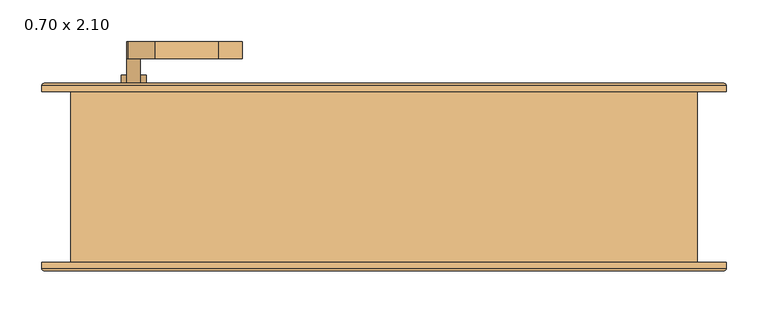
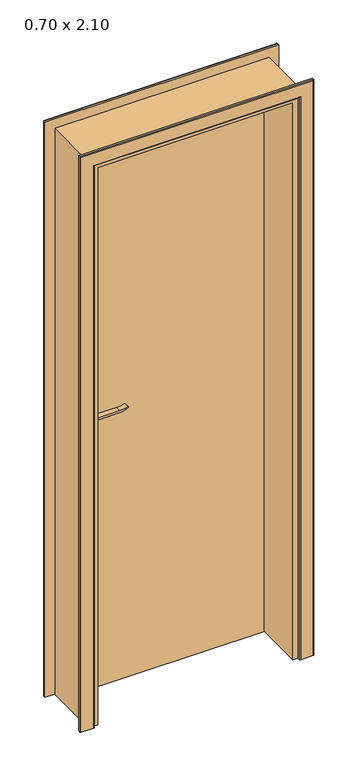
"""IFC4 building model written with IfcOpenShell, lengths in millimetres: door geometry, .CC_ND 300_PORTA SIMPLES DE ABRIR_COM EXTENSÃO : 0.70 x 2.10."""

import ifcopenshell
import ifcopenshell.guid

model = None  # the IFC model being written
_history = None  # IfcOwnerHistory: only IFC2X3 demands one
_inside = {}  # id of a spatial element -> (the spatial element, [elements in it])
_under = {}  # id of a project, library or spatial element -> (it, [spatial elements below it])
_declared = {}  # id of a project -> (the project, [libraries it declares])
_typed = {}  # id of a type object -> (the type object, [elements of that type])
_made_of = {}  # id of a material, layer set ... -> (it, [elements and type objects made of it])


def new_model(schema):
    """Start an empty IFC model of exactly this schema.

    Asked for "IFC4X3", IfcOpenShell would pick the latest addendum, in which some entities
    have other attributes; the version numbers below select the first issue.
    IFC2X3 requires an IfcOwnerHistory on every rooted entity: one is made here for all.
    """
    global model, _history
    if schema == "IFC4X3":
        model = ifcopenshell.file(schema_version=(4, 3, 0, 0))
    else:
        model = ifcopenshell.file(schema=schema)
    _inside.clear()
    _under.clear()
    _declared.clear()
    _typed.clear()
    _made_of.clear()
    _history = None
    if model.schema == "IFC2X3":
        org = make("IfcOrganization", Name="unknown")
        user = make(
            "IfcPersonAndOrganization",
            ThePerson=make("IfcPerson", FamilyName="unknown"),
            TheOrganization=org,
        )
        app = make(
            "IfcApplication",
            ApplicationDeveloper=org,
            Version="unknown",
            ApplicationFullName="unknown",
            ApplicationIdentifier="unknown",
        )
        _history = make(
            "IfcOwnerHistory",
            OwningUser=user,
            OwningApplication=app,
            ChangeAction="ADDED",
            CreationDate=0,
        )
    return model


def make(cls, **values):
    """One entity of the class cls with the attributes given. An attribute that is None is left unset."""
    return model.create_entity(
        cls, **{name: value for name, value in values.items() if value is not None}
    )


def rooted(cls, **values):
    """An entity with a GlobalId (a new one), such as an element, a storey or a relation."""
    return make(cls, GlobalId=ifcopenshell.guid.new(), OwnerHistory=_history, **values)


def si_unit(unit_type, name, prefix=None):
    """IfcSIUnit, for example si_unit("LENGTHUNIT", "METRE", prefix="MILLI")."""
    return make("IfcSIUnit", UnitType=unit_type, Prefix=prefix, Name=name)


def assignment(units):
    """IfcUnitAssignment: the units of a project."""
    return None if units is None else make("IfcUnitAssignment", Units=units)


def point(xyz):
    """IfcCartesianPoint."""
    return None if xyz is None else make("IfcCartesianPoint", Coordinates=xyz)


def direction(xyz):
    """IfcDirection."""
    return None if xyz is None else make("IfcDirection", DirectionRatios=xyz)


def frame(location, z_axis=None, x_axis=None):
    """IfcAxis2Placement3D, a coordinate frame: its origin and axes. An axis left out is left unset."""
    return make(
        "IfcAxis2Placement3D",
        Location=point(location),
        Axis=direction(z_axis),
        RefDirection=direction(x_axis),
    )


def frame_2d(location, x_axis=None):
    """IfcAxis2Placement2D, a coordinate frame in the plane: its origin and x axis."""
    return make(
        "IfcAxis2Placement2D", Location=point(location), RefDirection=direction(x_axis)
    )


def origin():
    """The frame at (0, 0, 0) with its axes left unset."""
    return frame((0.0, 0.0, 0.0))


def origin_with_axes():
    """The frame at (0, 0, 0) with the z axis (0, 0, 1) and the x axis (1, 0, 0) written out."""
    return frame((0.0, 0.0, 0.0), z_axis=(0.0, 0.0, 1.0), x_axis=(1.0, 0.0, 0.0))


def place(relative_to, where):
    """IfcLocalPlacement: puts the frame where relative to a parent placement (None: the world)."""
    return make(
        "IfcLocalPlacement", PlacementRelTo=relative_to, RelativePlacement=where
    )


def context(
    kind, dimensions, precision=None, world=None, true_north=None, identifier=None
):
    """IfcGeometricRepresentationContext, for example the 3D "Model" context."""
    return make(
        "IfcGeometricRepresentationContext",
        ContextIdentifier=identifier,
        ContextType=kind,
        CoordinateSpaceDimension=dimensions,
        Precision=precision,
        WorldCoordinateSystem=world,
        TrueNorth=true_north,
    )


def project(units=None, contexts=None):
    """IfcProject with its units and contexts."""
    return rooted(
        "IfcProject",
        Name="project",
        RepresentationContexts=contexts,
        UnitsInContext=assignment(units),
    )


def spatial(cls, under=None, at=None, **own):
    """A site, building, storey or space (cls), placed at a placement, below another one or the project."""
    s = rooted(cls, ObjectPlacement=at, **own)
    if under is not None:
        _under.setdefault(under.id(), (under, []))[1].append(s)
    return s


def polyline(points):
    """IfcPolyline through the points."""
    return make("IfcPolyline", Points=[point(p) for p in points])


def circle_curve(where, radius):
    """IfcCircle in the frame where."""
    return make("IfcCircle", Position=where, Radius=radius)


def ellipse_curve(where, semi_axis1, semi_axis2):
    """IfcEllipse in the frame where."""
    return make(
        "IfcEllipse", Position=where, SemiAxis1=semi_axis1, SemiAxis2=semi_axis2
    )


def trimmed(basis, trim1, trim2, sense, master):
    """IfcTrimmedCurve: the piece of a basis curve between two trims."""
    return make(
        "IfcTrimmedCurve",
        BasisCurve=basis,
        Trim1=trim1,
        Trim2=trim2,
        SenseAgreement=sense,
        MasterRepresentation=master,
    )


def segment(curve, same_sense, transition):
    """IfcCompositeCurveSegment."""
    return make(
        "IfcCompositeCurveSegment",
        Transition=transition,
        SameSense=same_sense,
        ParentCurve=curve,
    )


def composite_curve(segments, self_intersect=None):
    """IfcCompositeCurve: segments joined end to end."""
    return make("IfcCompositeCurve", Segments=segments, SelfIntersect=self_intersect)


def outline(outer, holes=None, kind="AREA"):
    """IfcArbitraryClosedProfileDef: a profile drawn as a closed curve; with holes, ...WithVoids."""
    if holes is None:
        return make("IfcArbitraryClosedProfileDef", ProfileType=kind, OuterCurve=outer)
    return make(
        "IfcArbitraryProfileDefWithVoids",
        ProfileType=kind,
        OuterCurve=outer,
        InnerCurves=holes,
    )


def extrude(swept, where, along, depth):
    """IfcExtrudedAreaSolid: the profile swept, set in the frame where, extruded along a direction by depth."""
    return make(
        "IfcExtrudedAreaSolid",
        SweptArea=swept,
        Position=where,
        ExtrudedDirection=direction(along),
        Depth=depth,
    )


def faces_of(points, faces, orient=None, outer=None):
    """IfcFace entities. A face is a list of loops; a loop is a list of indices into points, from 0.

    orient and outer hold one flag for each loop. By default every Orientation is true, the
    first loop of a face is its IfcFaceOuterBound and the others are IfcFaceBound.
    """
    made = []
    for i, loops in enumerate(faces):
        bounds = []
        for j, loop in enumerate(loops):
            is_outer = j == 0 if outer is None else outer[i][j]
            bounds.append(
                make(
                    "IfcFaceOuterBound" if is_outer else "IfcFaceBound",
                    Bound=make("IfcPolyLoop", Polygon=[points[k] for k in loop]),
                    Orientation=True if orient is None else orient[i][j],
                )
            )
        made.append(make("IfcFace", Bounds=bounds))
    return made


def faceted_brep(points, faces, orient=None, outer=None, voids=None):
    """IfcFacetedBrep: a solid bounded by flat faces; with voids (closed shells), ...WithVoids."""
    shared = [point(p) for p in points]
    hull = make("IfcClosedShell", CfsFaces=faces_of(shared, faces, orient, outer))
    if voids is None:
        return make("IfcFacetedBrep", Outer=hull)
    return make(
        "IfcFacetedBrepWithVoids",
        Outer=hull,
        Voids=[
            make(cls, CfsFaces=faces_of(shared, fs, o, b)) for cls, fs, o, b in voids
        ],
    )


def shape(context_of_items, identifier, shape_type, items):
    """IfcShapeRepresentation: the items that make up one representation, for example the "Body"."""
    return make(
        "IfcShapeRepresentation",
        ContextOfItems=context_of_items,
        RepresentationIdentifier=identifier,
        RepresentationType=shape_type,
        Items=items,
    )


def source(mapping_origin, context_of_items, identifier, shape_type, items):
    """IfcRepresentationMap: a shape defined once, which mapped items show again and again."""
    return make(
        "IfcRepresentationMap",
        MappingOrigin=mapping_origin,
        MappedRepresentation=shape(context_of_items, identifier, shape_type, items),
    )


def transform(
    local_origin,
    x_axis=None,
    y_axis=None,
    z_axis=None,
    scale=None,
    scale2=None,
    scale3=None,
    uniform=True,
):
    """IfcCartesianTransformationOperator3D, or its non-uniform kind. x_axis, y_axis, z_axis: its Axis1, 2, 3."""
    if uniform:
        return make(
            "IfcCartesianTransformationOperator3D",
            Axis1=direction(x_axis),
            Axis2=direction(y_axis),
            LocalOrigin=point(local_origin),
            Scale=scale,
            Axis3=direction(z_axis),
        )
    return make(
        "IfcCartesianTransformationOperator3DnonUniform",
        Axis1=direction(x_axis),
        Axis2=direction(y_axis),
        LocalOrigin=point(local_origin),
        Scale=scale,
        Axis3=direction(z_axis),
        Scale2=scale2,
        Scale3=scale3,
    )


def mapped(mapping_source, mapping_target):
    """IfcMappedItem: shows the shape of a source again, moved by a transform."""
    return make(
        "IfcMappedItem", MappingSource=mapping_source, MappingTarget=mapping_target
    )


def made_of(thing, what):
    """Note that an element or type object is made of a material, layer set ...; save() writes the relation."""
    if what is not None:
        _made_of.setdefault(what.id(), (what, []))[1].append(thing)
    return thing


def element(
    cls,
    number,
    at=None,
    inside=None,
    cuts=None,
    type_object=None,
    material=None,
    context=None,
    identifier="Body",
    shape_type=None,
    held_by="IfcProductDefinitionShape",
    body=None,
    shapes=None,
    **own,
):
    """One element of the class cls, such as IfcWall. Its Tag is "e" and its number.

    at: its placement. inside: the storey or other place that contains it. cuts: it is an
    opening in that element (IfcRelVoidsElement). A single representation is given by context,
    identifier, shape_type and body (its items); several are given by shapes. held_by: the class
    of the entity that holds the representations. save() writes the other relations.
    """
    e = rooted(cls, Tag="e%d" % number, ObjectPlacement=at, **own)
    if body is not None:
        shapes = [shape(context, identifier, shape_type, body)]
    if shapes is not None:
        e.Representation = make(held_by, Representations=shapes)
    if inside is not None:
        _inside.setdefault(inside.id(), (inside, []))[1].append(e)
    if cuts is not None:
        rooted(
            "IfcRelVoidsElement", RelatingBuildingElement=cuts, RelatedOpeningElement=e
        )
    if type_object is not None:
        _typed.setdefault(type_object.id(), (type_object, []))[1].append(e)
    return made_of(e, material)


def aggregate(whole, parts):
    """IfcRelAggregates: a whole, such as a stair, and the parts it consists of."""
    return rooted("IfcRelAggregates", RelatingObject=whole, RelatedObjects=parts)


def save(model, path):
    """Write the relations noted so far, then the file.

    IfcRelAggregates (storeys below a building ...), IfcRelContainedInSpatialStructure (elements
    in a storey), IfcRelDefinesByType, IfcRelAssociatesMaterial and IfcRelDeclares: one each for
    every whole, place, type object, material and project.
    """
    for whole, parts in _under.values():
        aggregate(whole, parts)
    for where, things in _inside.values():
        rooted(
            "IfcRelContainedInSpatialStructure",
            RelatedElements=things,
            RelatingStructure=where,
        )
    for kind, things in _typed.values():
        rooted("IfcRelDefinesByType", RelatedObjects=things, RelatingType=kind)
    for what, things in _made_of.values():
        rooted("IfcRelAssociatesMaterial", RelatedObjects=things, RelatingMaterial=what)
    for by, libraries in _declared.values():
        rooted("IfcRelDeclares", RelatingContext=by, RelatedDefinitions=libraries)
    model.write(path)


def plane_surface(at):
    """IfcPlane: the flat surface through the origin of the frame at, square to its z axis."""
    return make("IfcPlane", Position=at)


def cylinder_surface(at, radius):
    """IfcCylindricalSurface: all points at the distance radius from the z axis of the frame at."""
    return make("IfcCylindricalSurface", Position=at, Radius=radius)


def advanced_brep(points, edges, surfaces, faces):
    """IfcAdvancedBrep: a solid bounded by faces that lie on surfaces and meet in shared edges.

    An edge is (start, end): straight between two places in points (the first is 0);
    or (start, end, curve); or (start, end, curve, False) where it runs against its curve.
    A face is (place in surfaces, loops), or (place, loops, False) where it looks against
    its surface's normal. A loop lists edges by number (the first is 1), with a minus sign
    where the edge is run from its end to its start. The first loop is the outer one.
    """
    corners = [point(p) for p in points]
    vertices = [make("IfcVertexPoint", VertexGeometry=c) for c in corners]
    made = []
    for start, end, *more in edges:
        made.append(
            make(
                "IfcEdgeCurve",
                EdgeStart=vertices[start],
                EdgeEnd=vertices[end],
                EdgeGeometry=more[0] if more else make("IfcPolyline", Points=[corners[start], corners[end]]),
                SameSense=more[1] if len(more) > 1 else True,
            )
        )
    hull = []
    for where, loops, *sense in faces:
        bounds = []
        for j, loop in enumerate(loops):
            ring = [make("IfcOrientedEdge", EdgeElement=made[abs(k) - 1], Orientation=k > 0) for k in loop]
            bounds.append(
                make(
                    "IfcFaceOuterBound" if j == 0 else "IfcFaceBound",
                    Bound=make("IfcEdgeLoop", EdgeList=ring),
                    Orientation=True,
                )
            )
        hull.append(make("IfcAdvancedFace", Bounds=bounds, FaceSurface=surfaces[where], SameSense=sense[0] if sense else True))
    return make("IfcAdvancedBrep", Outer=make("IfcClosedShell", CfsFaces=hull))


def door_0_70_x_2_10_01854108(model_context):
    return source(origin(), model_context, "Body", "SolidModel", [
        extrude(outline(composite_curve([segment(trimmed(circle_curve(frame_2d((964.5, -300.0)), 15.0), [point((964.5, -285.0))], [point((964.5, -315.0))], False, "CARTESIAN"), True, "CONTINUOUS"), segment(trimmed(circle_curve(frame_2d((964.5, -300.0)), 15.0), [point((964.5, -315.0))], [point((964.5, -285.0))], False, "CARTESIAN"), True, "CONTINUOUS")], self_intersect=False)), frame((0.0, 127.9, 0.0), z_axis=(0.0, 1.0, 0.0), x_axis=(0.0, 0.0, 1.0)), (0.0, 0.0, 1.0), 10.0),
        extrude(outline(composite_curve([segment(trimmed(circle_curve(frame_2d((964.5, -300.0)), 15.0), [point((964.5, -285.0))], [point((964.5, -315.0))], False, "CARTESIAN"), True, "CONTINUOUS"), segment(trimmed(circle_curve(frame_2d((964.5, -300.0)), 15.0), [point((964.5, -315.0))], [point((964.5, -285.0))], False, "CARTESIAN"), True, "CONTINUOUS")], self_intersect=False)), frame((0.0, 67.9, 0.0), z_axis=(0.0, 1.0, 0.0), x_axis=(0.0, 0.0, 1.0)), (0.0, 0.0, 1.0), 10.0),
        extrude(outline(composite_curve([segment(trimmed(circle_curve(frame_2d((1024.5, -300.0)), 8.0), [point((1029.1523287, -306.5081363))], [point((1024.5, -292.0))], False, "CARTESIAN"), True, "CONTINUOUS"), segment(trimmed(circle_curve(frame_2d((1019.3738613, -274.6138099)), 18.1261387), [point((1024.5, -292.0))], [point((1037.5, -274.6138099))], True, "CARTESIAN"), True, "CONTINUOUS"), segment(polyline([(1037.5, -274.6138099), (1037.5, -198.3564091)]), True, "CONTINUOUS"), segment(trimmed(circle_curve(frame_2d((1096.7709207, -201.9396612)), 59.3791355), [point((1037.5, -198.3564091))], [point((1046.7135558, -170.0))], False, "CARTESIAN"), True, "CONTINUOUS"), segment(polyline([(1046.7135558, -170.0), (1049.5, -170.0)]), True, "CONTINUOUS"), segment(trimmed(circle_curve(frame_2d((1127.7850638, -198.4227909)), 83.2850902), [point((1049.5, -170.0))], [point((1044.5, -198.3564091))], True, "CARTESIAN"), True, "CONTINUOUS"), segment(polyline([(1044.5, -198.3564091), (1044.5, -274.6325667)]), True, "CONTINUOUS"), segment(trimmed(circle_curve(frame_2d((1007.2555521, -276.3324871)), 37.2832219), [point((1044.5, -274.6325667))], [point((1029.1523287, -306.5081363))], False, "CARTESIAN"), True, "CONTINUOUS")], self_intersect=False)), frame((0.0, 157.9, 0.0), z_axis=(0.0, 1.0, 0.0), x_axis=(0.0, 0.0, 1.0)), (0.0, 0.0, 1.0), 20.0),
        extrude(outline(composite_curve([segment(trimmed(circle_curve(frame_2d((1019.3738682, -274.6138122)), 18.1261318), [point((1024.4999903, -292.0))], [point((1037.5, -274.6138122))], True, "CARTESIAN"), True, "CONTINUOUS"), segment(polyline([(1037.5, -274.6138122), (1037.5, -198.3564091)]), True, "CONTINUOUS"), segment(trimmed(circle_curve(frame_2d((1096.7709207, -201.9396612)), 59.3791355), [point((1037.5, -198.3564091))], [point((1046.7135558, -170.0))], False, "CARTESIAN"), True, "CONTINUOUS"), segment(polyline([(1046.7135558, -170.0), (1049.5, -170.0)]), True, "CONTINUOUS"), segment(trimmed(circle_curve(frame_2d((1127.7850638, -198.4227909)), 83.2850902), [point((1049.5, -170.0))], [point((1044.5, -198.3564091))], True, "CARTESIAN"), True, "CONTINUOUS"), segment(polyline([(1044.5, -198.3564091), (1044.5, -274.6325667)]), True, "CONTINUOUS"), segment(trimmed(circle_curve(frame_2d((1007.2555521, -276.3324871)), 37.2832219), [point((1044.5, -274.6325667))], [point((1029.1523287, -306.5081363))], False, "CARTESIAN"), True, "CONTINUOUS"), segment(trimmed(circle_curve(frame_2d((1024.5, -300.0)), 8.0), [point((1029.1523287, -306.5081363))], [point((1024.4999903, -292.0))], False, "CARTESIAN"), True, "CONTINUOUS")], self_intersect=False)), frame((0.0, 27.9, 0.0), z_axis=(0.0, 1.0, 0.0), x_axis=(0.0, 0.0, 1.0)), (0.0, 0.0, 1.0), 20.0),
        extrude(outline(composite_curve([segment(trimmed(circle_curve(frame_2d((1024.5, -300.0)), 8.0), [point((1024.5, -292.0))], [point((1024.5, -308.0))], False, "CARTESIAN"), True, "CONTINUOUS"), segment(trimmed(circle_curve(frame_2d((1024.5, -300.0)), 8.0), [point((1024.5, -308.0))], [point((1024.5, -292.0))], False, "CARTESIAN"), True, "CONTINUOUS")], self_intersect=False)), frame((0.0, 127.9, 0.0), z_axis=(0.0, 1.0, 0.0), x_axis=(0.0, 0.0, 1.0)), (0.0, 0.0, 1.0), 30.0),
        extrude(outline(composite_curve([segment(trimmed(circle_curve(frame_2d((1024.5, -300.0)), 8.0), [point((1024.5, -292.0))], [point((1024.5, -308.0))], False, "CARTESIAN"), True, "CONTINUOUS"), segment(trimmed(circle_curve(frame_2d((1024.5, -300.0)), 8.0), [point((1024.5, -308.0))], [point((1024.5, -292.0))], False, "CARTESIAN"), True, "CONTINUOUS")], self_intersect=False)), frame((0.0, 47.9, 0.0), z_axis=(0.0, 1.0, 0.0), x_axis=(0.0, 0.0, 1.0)), (0.0, 0.0, 1.0), 30.0),
        extrude(outline(composite_curve([segment(trimmed(circle_curve(frame_2d((954.5, -300.0)), 25.0), [point((954.5, -325.0))], [point((954.5, -275.0))], False, "CARTESIAN"), True, "CONTINUOUS"), segment(polyline([(954.5, -275.0), (1024.5, -275.0)]), True, "CONTINUOUS"), segment(trimmed(circle_curve(frame_2d((1024.5, -300.0)), 25.0), [point((1024.5, -275.0))], [point((1024.5, -325.0))], False, "CARTESIAN"), True, "CONTINUOUS"), segment(polyline([(1024.5, -325.0), (954.5, -325.0)]), True, "CONTINUOUS")], self_intersect=False)), frame((0.0, 117.9, 0.0), z_axis=(0.0, 1.0, 0.0), x_axis=(0.0, 0.0, 1.0)), (0.0, 0.0, 1.0), 10.0),
        extrude(outline(composite_curve([segment(trimmed(circle_curve(frame_2d((954.5, -300.0)), 25.0), [point((954.5, -325.0))], [point((954.5, -275.0))], False, "CARTESIAN"), True, "CONTINUOUS"), segment(polyline([(954.5, -275.0), (1024.5, -275.0)]), True, "CONTINUOUS"), segment(trimmed(circle_curve(frame_2d((1024.5, -300.0)), 25.0), [point((1024.5, -275.0))], [point((1024.5, -325.0))], False, "CARTESIAN"), True, "CONTINUOUS"), segment(polyline([(1024.5, -325.0), (954.5, -325.0)]), True, "CONTINUOUS")], self_intersect=False)), frame((0.0, 77.9, 0.0), z_axis=(0.0, 1.0, 0.0), x_axis=(0.0, 0.0, 1.0)), (0.0, 0.0, 1.0), 10.0),
        advanced_brep(
        [(-410.0, 117.9, 0.0), (-410.0, 124.9, 0.0), (-407.0, 127.9, 0.0), (-363.0, 127.9, 0.0), (-360.0, 124.9, 0.0), (-360.0, 117.9, 0.0), (-360.0, 117.9, 2085.0), (360.0, 117.9, 2085.0), (360.0, 117.9, 0.0), (410.0, 117.9, 0.0), (410.0, 117.9, 2135.0), (-410.0, 117.9, 2135.0), (-360.0, 124.9, 2085.0), (-363.0, 127.9, 2088.0), (-407.0, 127.9, 2132.0), (407.0, 127.9, 2132.0), (407.0, 127.9, 0.0), (363.0, 127.9, 0.0), (363.0, 127.9, 2088.0), (-410.0, 124.9, 2135.0), (410.0, 124.9, 0.0), (410.0, 124.9, 2135.0), (360.0, 124.9, 0.0), (360.0, 124.9, 2085.0)],
        [
            (0, 1),
            (1, 2, circle_curve(frame((-407.0, 124.9, 0.0), z_axis=(0.0, 0.0, -1.0), x_axis=(1.0, 0.0, 0.0)), 3.0)),
            (2, 3),
            (3, 4, circle_curve(frame((-363.0, 124.9, 0.0), z_axis=(0.0, 0.0, -1.0), x_axis=(1.0, 0.0, 0.0)), 3.0)),
            (4, 5),
            (5, 0),
            (5, 6),
            (6, 7),
            (7, 8),
            (8, 9),
            (9, 10),
            (10, 11),
            (11, 0),
            (4, 12),
            (12, 6),
            (3, 13),
            (13, 12, ellipse_curve(frame((-363.0, 124.9, 2088.0), z_axis=(-0.7071067811865475, 0.0, -0.7071067811865475), x_axis=(0.7071067811865474, 0.0, -0.7071067811865476)), 4.2426407, 3.0)),
            (2, 14),
            (14, 15),
            (15, 16),
            (16, 17),
            (17, 18),
            (18, 13),
            (1, 19),
            (19, 14, ellipse_curve(frame((-407.0, 124.9, 2132.0), z_axis=(-0.7071067811865475, 0.0, -0.7071067811865475), x_axis=(0.7071067811865474, 0.0, -0.7071067811865476)), 4.2426407, 3.0)),
            (11, 19),
            (9, 20),
            (20, 21),
            (21, 10),
            (8, 22),
            (22, 17, circle_curve(frame((363.0, 124.9, 0.0), z_axis=(0.0, 0.0, -1.0), x_axis=(-1.0, 0.0, 0.0)), 3.0)),
            (16, 20, circle_curve(frame((407.0, 124.9, 0.0), z_axis=(0.0, 0.0, -1.0), x_axis=(-1.0, 0.0, 0.0)), 3.0)),
            (23, 22),
            (7, 23),
            (23, 18, ellipse_curve(frame((363.0, 124.9, 2088.0), z_axis=(0.7071067811865475, 0.0, -0.7071067811865475), x_axis=(0.7071067811865474, 0.0, 0.7071067811865476)), 4.2426407, 3.0)),
            (15, 21, ellipse_curve(frame((407.0, 124.9, 2132.0), z_axis=(0.7071067811865475, 0.0, -0.7071067811865475), x_axis=(0.7071067811865474, 0.0, 0.7071067811865476)), 4.2426407, 3.0)),
            (12, 23),
            (21, 19),
        ],
        [
            plane_surface(frame((-360.0, 117.9, 0.0), z_axis=(0.0, 0.0, -1.0), x_axis=(0.0, -1.0, 0.0))),
            plane_surface(frame((-410.0, 117.9, 0.0), z_axis=(0.0, -1.0, 0.0), x_axis=(0.0, 0.0, 1.0))),
            plane_surface(frame((-360.0, 117.9, 0.0), z_axis=(1.0, 0.0, 0.0), x_axis=(0.0, 0.0, 1.0))),
            cylinder_surface(frame((-363.0, 124.9, 0.0), z_axis=(0.0, 0.0, -1.0), x_axis=(1.0, 0.0, 0.0)), 3.0),
            plane_surface(frame((-363.0, 127.9, 0.0), z_axis=(0.0, 1.0, 0.0), x_axis=(0.0, 0.0, 1.0))),
            cylinder_surface(frame((-407.0, 124.9, 0.0), z_axis=(0.0, 0.0, -1.0), x_axis=(1.0, 0.0, 0.0)), 3.0),
            plane_surface(frame((-410.0, 124.9, 0.0), z_axis=(-1.0, 0.0, 0.0), x_axis=(0.0, 0.0, 1.0))),
            plane_surface(frame((410.0, 124.9, 2135.0), z_axis=(1.0, 0.0, 0.0), x_axis=(0.0, 0.0, -1.0))),
            plane_surface(frame((360.0, 117.9, 0.0), z_axis=(0.0, 0.0, -1.0), x_axis=(0.0, -1.0, 0.0))),
            plane_surface(frame((360.0, 117.9, 2085.0), z_axis=(-1.0, 0.0, 0.0), x_axis=(0.0, 0.0, -1.0))),
            cylinder_surface(frame((363.0, 124.9, 2085.0), z_axis=(0.0, 0.0, 1.0), x_axis=(-1.0, 0.0, 0.0)), 3.0),
            cylinder_surface(frame((407.0, 124.9, 2085.0), z_axis=(0.0, 0.0, 1.0), x_axis=(-1.0, 0.0, 0.0)), 3.0),
            plane_surface(frame((-360.0, 117.9, 2085.0), z_axis=(0.0, 0.0, -1.0), x_axis=(1.0, 0.0, 0.0))),
            plane_surface(frame((-410.0, 124.9, 2135.0), z_axis=(0.0, 0.0, 1.0), x_axis=(1.0, 0.0, 0.0))),
            cylinder_surface(frame((-360.0, 124.9, 2088.0), z_axis=(-1.0, 0.0, 0.0), x_axis=(0.0, 0.0, -1.0)), 3.0),
            cylinder_surface(frame((-360.0, 124.9, 2132.0), z_axis=(-1.0, 0.0, 0.0), x_axis=(0.0, 0.0, -1.0)), 3.0),
        ],
        [
            (0, [[1, 2, 3, 4, 5, 6]]),
            (1, [[7, 8, 9, 10, 11, 12, 13, -6]]),
            (2, [[14, 15, -7, -5]]),
            (3, [[16, 17, -14, -4]]),
            (4, [[18, 19, 20, 21, 22, 23, -16, -3]]),
            (5, [[24, 25, -18, -2]]),
            (6, [[-13, 26, -24, -1]]),
            (7, [[-11, 27, 28, 29]]),
            (8, [[-10, 30, 31, -21, 32, -27]]),
            (9, [[33, -30, -9, 34]]),
            (10, [[-22, -31, -33, 35]]),
            (11, [[-28, -32, -20, 36]]),
            (12, [[37, -34, -8, -15]]),
            (13, [[-12, -29, 38, -26]]),
            (14, [[-23, -35, -37, -17]]),
            (15, [[-38, -36, -19, -25]]),
        ],
    ),
        advanced_brep(
        [(410.0, -86.9, 0.0), (410.0, -93.9342217, 0.0), (407.0342217, -96.9, 0.0), (362.9842717, -96.9, 0.0), (360.0, -93.9157283, 0.0), (360.0, -86.9, 0.0), (360.0, -86.9, 2085.0), (-360.0, -86.9, 2085.0), (-360.0, -86.9, 0.0), (-410.0, -86.9, 0.0), (-410.0, -86.9, 2135.0), (410.0, -86.9, 2135.0), (360.0, -93.9157283, 2085.0), (362.9842717, -96.9, 2087.9842717), (407.0342217, -96.9, 2132.0342217), (-407.0342217, -96.9, 2132.0342217), (-407.0342217, -96.9, 0.0), (-362.9842717, -96.9, 0.0), (-362.9842717, -96.9, 2087.9842717), (410.0, -93.9342217, 2135.0), (-410.0, -93.9342217, 0.0), (-410.0, -93.9342217, 2135.0), (-360.0, -93.9157283, 0.0), (-360.0, -93.9157283, 2085.0)],
        [
            (0, 1),
            (1, 2, circle_curve(frame((407.0342217, -93.9342217, 0.0), z_axis=(0.0, 0.0, -1.0), x_axis=(1.0, 0.0, 0.0)), 2.9657783)),
            (2, 3),
            (3, 4, circle_curve(frame((362.9842717, -93.9157283, 0.0), z_axis=(0.0, 0.0, -1.0), x_axis=(1.0, 0.0, 0.0)), 2.9842717)),
            (4, 5),
            (5, 0),
            (5, 6),
            (6, 7),
            (7, 8),
            (8, 9),
            (9, 10),
            (10, 11),
            (11, 0),
            (4, 12),
            (12, 6),
            (3, 13),
            (13, 12, ellipse_curve(frame((362.9842717, -93.9157283, 2087.9842717), z_axis=(0.7071067811865475, 0.0, -0.7071067811865475), x_axis=(-0.7071067811865474, 0.0, -0.7071067811865476)), 4.2203975, 2.9842717)),
            (2, 14),
            (14, 15),
            (15, 16),
            (16, 17),
            (17, 18),
            (18, 13),
            (1, 19),
            (19, 14, ellipse_curve(frame((407.0342217, -93.9342217, 2132.0342217), z_axis=(0.7071067811865475, 0.0, -0.7071067811865475), x_axis=(-0.7071067811865474, 0.0, -0.7071067811865476)), 4.1942438, 2.9657783)),
            (11, 19),
            (9, 20),
            (20, 21),
            (21, 10),
            (8, 22),
            (22, 17, circle_curve(frame((-362.9842717, -93.9157283, 0.0), z_axis=(0.0, 0.0, -1.0), x_axis=(-1.0, 0.0, 0.0)), 2.9842717)),
            (16, 20, circle_curve(frame((-407.0342217, -93.9342217, 0.0), z_axis=(0.0, 0.0, -1.0), x_axis=(-1.0, 0.0, 0.0)), 2.9657783)),
            (23, 22),
            (7, 23),
            (23, 18, ellipse_curve(frame((-362.9842717, -93.9157283, 2087.9842717), z_axis=(-0.7071067811865475, 0.0, -0.7071067811865475), x_axis=(-0.7071067811865474, 0.0, 0.7071067811865476)), 4.2203975, 2.9842717)),
            (15, 21, ellipse_curve(frame((-407.0342217, -93.9342217, 2132.0342217), z_axis=(-0.7071067811865475, 0.0, -0.7071067811865475), x_axis=(-0.7071067811865474, 0.0, 0.7071067811865476)), 4.1942438, 2.9657783)),
            (12, 23),
            (21, 19),
        ],
        [
            plane_surface(frame((360.0, -86.9, 0.0), z_axis=(0.0, 0.0, -1.0), x_axis=(0.0, -1.0, 0.0))),
            plane_surface(frame((410.0, -86.9, 0.0), z_axis=(0.0, 1.0, 0.0), x_axis=(0.0, 0.0, 1.0))),
            plane_surface(frame((360.0, -86.9, 0.0), z_axis=(-1.0, 0.0, 0.0), x_axis=(0.0, 0.0, 1.0))),
            cylinder_surface(frame((362.9842717, -93.9157283, 0.0), z_axis=(0.0, 0.0, -1.0), x_axis=(1.0, 0.0, 0.0)), 2.9842717),
            plane_surface(frame((362.9842717, -96.9, 0.0), z_axis=(0.0, -1.0, 0.0), x_axis=(0.0, 0.0, 1.0))),
            cylinder_surface(frame((407.0342217, -93.9342217, 0.0), z_axis=(0.0, 0.0, -1.0), x_axis=(1.0, 0.0, 0.0)), 2.9657783),
            plane_surface(frame((410.0, -93.9342217, 0.0), z_axis=(1.0, 0.0, 0.0), x_axis=(0.0, 0.0, 1.0))),
            plane_surface(frame((-410.0, -93.9342217, 2135.0), z_axis=(-1.0, 0.0, 0.0), x_axis=(0.0, 0.0, -1.0))),
            plane_surface(frame((-360.0, -86.9, 0.0), z_axis=(0.0, 0.0, -1.0), x_axis=(0.0, -1.0, 0.0))),
            plane_surface(frame((-360.0, -86.9, 2085.0), z_axis=(1.0, 0.0, 0.0), x_axis=(0.0, 0.0, -1.0))),
            cylinder_surface(frame((-362.9842717, -93.9157283, 2085.0), z_axis=(0.0, 0.0, 1.0), x_axis=(-1.0, 0.0, 0.0)), 2.9842717),
            cylinder_surface(frame((-407.0342217, -93.9342217, 2085.0), z_axis=(0.0, 0.0, 1.0), x_axis=(-1.0, 0.0, 0.0)), 2.9657783),
            plane_surface(frame((360.0, -86.9, 2085.0), z_axis=(0.0, 0.0, -1.0), x_axis=(-1.0, 0.0, 0.0))),
            plane_surface(frame((410.0, -93.9342217, 2135.0), z_axis=(0.0, 0.0, 1.0), x_axis=(-1.0, 0.0, 0.0))),
            cylinder_surface(frame((360.0, -93.9157283, 2087.9842717), z_axis=(1.0, 0.0, 0.0), x_axis=(0.0, 0.0, 1.0)), 2.9842717),
            cylinder_surface(frame((360.0, -93.9342217, 2132.0342217), z_axis=(1.0, 0.0, 0.0), x_axis=(0.0, 0.0, 1.0)), 2.9657783),
        ],
        [
            (0, [[1, 2, 3, 4, 5, 6]]),
            (1, [[7, 8, 9, 10, 11, 12, 13, -6]]),
            (2, [[14, 15, -7, -5]]),
            (3, [[16, 17, -14, -4]]),
            (4, [[18, 19, 20, 21, 22, 23, -16, -3]]),
            (5, [[24, 25, -18, -2]]),
            (6, [[-13, 26, -24, -1]]),
            (7, [[-11, 27, 28, 29]]),
            (8, [[-10, 30, 31, -21, 32, -27]]),
            (9, [[33, -30, -9, 34]]),
            (10, [[-22, -31, -33, 35]]),
            (11, [[-28, -32, -20, 36]]),
            (12, [[37, -34, -8, -15]]),
            (13, [[-12, -29, 38, -26]]),
            (14, [[-23, -35, -37, -17]]),
            (15, [[-38, -36, -19, -25]]),
        ],
    ),
        faceted_brep([(342.0, -86.9, 0.0), (342.0, 87.9, 0.0), (350.0, 87.9, 0.0), (350.0, 117.9, 0.0), (375.0, 117.9, 0.0), (375.0, -86.9, 0.0), (375.0, -86.9, 2100.0), (-375.0, -86.9, 2100.0), (-375.0, -86.9, 0.0), (-342.0, -86.9, 0.0), (-342.0, -86.9, 2067.0), (342.0, -86.9, 2067.0), (375.0, 117.9, 2100.0), (350.0, 117.9, 2075.0), (-350.0, 117.9, 2075.0), (-350.0, 117.9, 0.0), (-375.0, 117.9, 0.0), (-375.0, 117.9, 2100.0), (350.0, 87.9, 2075.0), (342.0, 87.9, 2067.0), (-342.0, 87.9, 2067.0), (-342.0, 87.9, 0.0), (-350.0, 87.9, 0.0), (-350.0, 87.9, 2075.0)], [[[0, 1, 2, 3, 4, 5]], [[5, 6, 7, 8, 9, 10, 11, 0]], [[4, 12, 6, 5]], [[3, 13, 14, 15, 16, 17, 12, 4]], [[2, 18, 13, 3]], [[1, 19, 20, 21, 22, 23, 18, 2]], [[0, 11, 19, 1]], [[10, 9, 21, 20]], [[9, 8, 16, 15, 22, 21]], [[17, 16, 8, 7]], [[23, 22, 15, 14]], [[12, 17, 7, 6]], [[18, 23, 14, 13]], [[11, 10, 20, 19]]]),
        extrude(outline(polyline([(-350.0, 87.9), (-350.0, 117.9), (350.0, 117.9), (350.0, 87.9), (-350.0, 87.9)])), origin_with_axes(), (0.0, 0.0, 1.0), 2075.0),
    ])


if __name__ == "__main__":
    model = new_model("IFC4")
    model_context = context("Model", 3, world=origin())
    ifc_project = project(units=[si_unit("LENGTHUNIT", "METRE", prefix="MILLI")], contexts=[model_context])
    site = spatial("IfcSite", under=ifc_project)
    building = spatial("IfcBuilding", under=site)
    placement = place(None, origin())
    door_0_70_x_2_10_shape = door_0_70_x_2_10_01854108(model_context)
    element("IfcDoor", 1, ObjectType=".CC_ND 300_PORTA SIMPLES DE ABRIR_COM EXTENSÃO : 0.70 x 2.10", at=placement, inside=building, context=model_context, shape_type="MappedRepresentation", body=[
        mapped(door_0_70_x_2_10_shape, transform((0.0, 0.0, 0.0), x_axis=(1.0, 0.0, 0.0), y_axis=(0.0, 1.0, 0.0), z_axis=(0.0, 0.0, 1.0))),
    ])
    save(model, "model.ifc")

# Revit data of these elements
# Type ".CC_ND 300_PORTA SIMPLES DE ABRIR_COM EXTENSÃO : 0.70 x 2.10"
#   Type Mark = "155"
#   Rough Width = 0.75 m
#   Espessura moldura externa = 0.01 m
#   Espessura moldura interna = 0.01 m
#   Largura moldura = 0.05 m
#   Extensão acabamento exterior [instance default] = 0.00 m
#   Extensão acabamento interior [instance default] = 0.00 m
#   Espessura batente = 0.025 m
#   Thickness = 0.03 m
#   Altura batente = 2.085 m
#   Aux Arco [instance default] = 0.70 m
#   Rough Height = 2.125 m
#   Height = 2.10 m
#   Width = 0.70 m
#   Moldura interna [instance default] = yes
#   Moldura externa [instance default] = yes
#   Porta = .MADEIRA COM PINTURA ESMALTE BRANCO ACETINADO
#   Moldura = .MADEIRA COM PINTURA ESMALTE BRANCO ACETINADO
#   Maçaneta = .ALUMÍNIO
#   Batente = .MADEIRA COM PINTURA ESMALTE BRANCO ACETINADO
#   Function = (empty or 0)
#   Wall Closure = (empty or 0)
# Element 1 (IfcDoor, ".CC_ND 300_PORTA SIMPLES DE ABRIR_COM EXTENSÃO : 0.70 x 2.10")
#   Extensão acabamento interior = 0.031 m
#   Aux Arco = 0.731 m
#   Materials on its faces: ".MADEIRA COM PINTURA ESMALTE BRANCO ACETINADO", ".ALUMÍNIO"
# Materials
#   ".MADEIRA COM PINTURA ESMALTE BRANCO ACETINADO": class ".CC_MADEIRAS", colour RGB 240 240 240, transparency 0, Description = "Madeira com pintura esmalte branco acetinado.", Cost = 0
#   ".ALUMÍNIO": class "CC_METAIS", colour RGB 244 244 244, transparency 0, Description = "Material alumínio", Cost = 0
